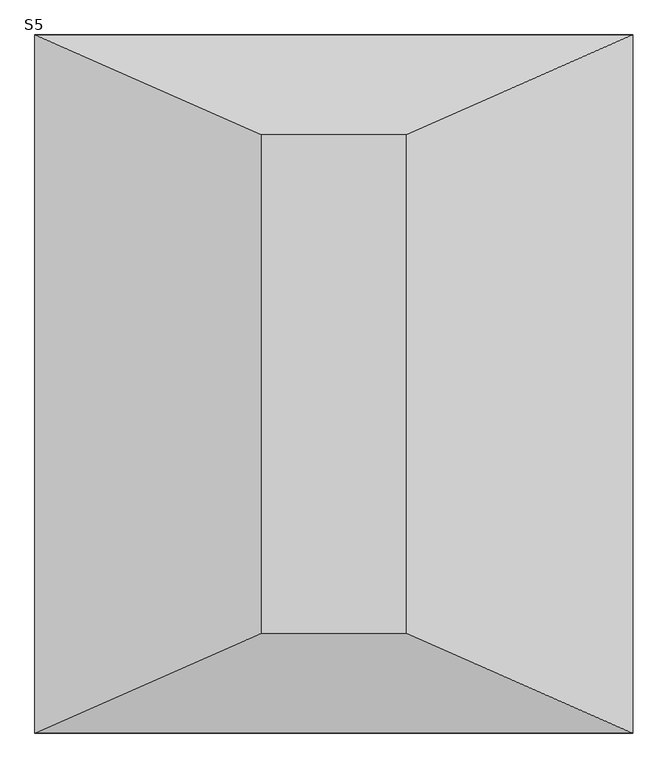
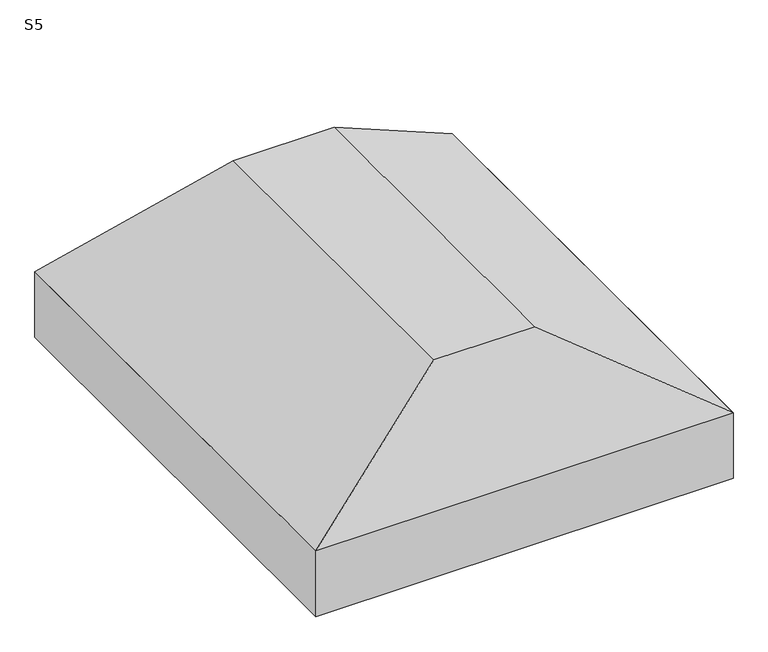
"""IFC4 building model written with IfcOpenShell, lengths in millimetres: fastener geometry, TQS - Sapata : S5."""

import ifcopenshell
import ifcopenshell.guid

model = None  # the IFC model being written
_history = None  # IfcOwnerHistory: only IFC2X3 demands one
_inside = {}  # id of a spatial element -> (the spatial element, [elements in it])
_under = {}  # id of a project, library or spatial element -> (it, [spatial elements below it])
_declared = {}  # id of a project -> (the project, [libraries it declares])
_typed = {}  # id of a type object -> (the type object, [elements of that type])
_made_of = {}  # id of a material, layer set ... -> (it, [elements and type objects made of it])


def new_model(schema):
    """Start an empty IFC model of exactly this schema.

    Asked for "IFC4X3", IfcOpenShell would pick the latest addendum, in which some entities
    have other attributes; the version numbers below select the first issue.
    IFC2X3 requires an IfcOwnerHistory on every rooted entity: one is made here for all.
    """
    global model, _history
    if schema == "IFC4X3":
        model = ifcopenshell.file(schema_version=(4, 3, 0, 0))
    else:
        model = ifcopenshell.file(schema=schema)
    _inside.clear()
    _under.clear()
    _declared.clear()
    _typed.clear()
    _made_of.clear()
    _history = None
    if model.schema == "IFC2X3":
        org = make("IfcOrganization", Name="unknown")
        user = make(
            "IfcPersonAndOrganization",
            ThePerson=make("IfcPerson", FamilyName="unknown"),
            TheOrganization=org,
        )
        app = make(
            "IfcApplication",
            ApplicationDeveloper=org,
            Version="unknown",
            ApplicationFullName="unknown",
            ApplicationIdentifier="unknown",
        )
        _history = make(
            "IfcOwnerHistory",
            OwningUser=user,
            OwningApplication=app,
            ChangeAction="ADDED",
            CreationDate=0,
        )
    return model


def make(cls, **values):
    """One entity of the class cls with the attributes given. An attribute that is None is left unset."""
    return model.create_entity(
        cls, **{name: value for name, value in values.items() if value is not None}
    )


def rooted(cls, **values):
    """An entity with a GlobalId (a new one), such as an element, a storey or a relation."""
    return make(cls, GlobalId=ifcopenshell.guid.new(), OwnerHistory=_history, **values)


def si_unit(unit_type, name, prefix=None):
    """IfcSIUnit, for example si_unit("LENGTHUNIT", "METRE", prefix="MILLI")."""
    return make("IfcSIUnit", UnitType=unit_type, Prefix=prefix, Name=name)


def assignment(units):
    """IfcUnitAssignment: the units of a project."""
    return None if units is None else make("IfcUnitAssignment", Units=units)


def point(xyz):
    """IfcCartesianPoint."""
    return None if xyz is None else make("IfcCartesianPoint", Coordinates=xyz)


def direction(xyz):
    """IfcDirection."""
    return None if xyz is None else make("IfcDirection", DirectionRatios=xyz)


def frame(location, z_axis=None, x_axis=None):
    """IfcAxis2Placement3D, a coordinate frame: its origin and axes. An axis left out is left unset."""
    return make(
        "IfcAxis2Placement3D",
        Location=point(location),
        Axis=direction(z_axis),
        RefDirection=direction(x_axis),
    )


def origin():
    """The frame at (0, 0, 0) with its axes left unset."""
    return frame((0.0, 0.0, 0.0))


def place(relative_to, where):
    """IfcLocalPlacement: puts the frame where relative to a parent placement (None: the world)."""
    return make(
        "IfcLocalPlacement", PlacementRelTo=relative_to, RelativePlacement=where
    )


def context(
    kind, dimensions, precision=None, world=None, true_north=None, identifier=None
):
    """IfcGeometricRepresentationContext, for example the 3D "Model" context."""
    return make(
        "IfcGeometricRepresentationContext",
        ContextIdentifier=identifier,
        ContextType=kind,
        CoordinateSpaceDimension=dimensions,
        Precision=precision,
        WorldCoordinateSystem=world,
        TrueNorth=true_north,
    )


def project(units=None, contexts=None):
    """IfcProject with its units and contexts."""
    return rooted(
        "IfcProject",
        Name="project",
        RepresentationContexts=contexts,
        UnitsInContext=assignment(units),
    )


def spatial(cls, under=None, at=None, **own):
    """A site, building, storey or space (cls), placed at a placement, below another one or the project."""
    s = rooted(cls, ObjectPlacement=at, **own)
    if under is not None:
        _under.setdefault(under.id(), (under, []))[1].append(s)
    return s


def polyline(points):
    """IfcPolyline through the points."""
    return make("IfcPolyline", Points=[point(p) for p in points])


def outline(outer, holes=None, kind="AREA"):
    """IfcArbitraryClosedProfileDef: a profile drawn as a closed curve; with holes, ...WithVoids."""
    if holes is None:
        return make("IfcArbitraryClosedProfileDef", ProfileType=kind, OuterCurve=outer)
    return make(
        "IfcArbitraryProfileDefWithVoids",
        ProfileType=kind,
        OuterCurve=outer,
        InnerCurves=holes,
    )


def extrude(swept, where, along, depth):
    """IfcExtrudedAreaSolid: the profile swept, set in the frame where, extruded along a direction by depth."""
    return make(
        "IfcExtrudedAreaSolid",
        SweptArea=swept,
        Position=where,
        ExtrudedDirection=direction(along),
        Depth=depth,
    )


def faces_of(points, faces, orient=None, outer=None):
    """IfcFace entities. A face is a list of loops; a loop is a list of indices into points, from 0.

    orient and outer hold one flag for each loop. By default every Orientation is true, the
    first loop of a face is its IfcFaceOuterBound and the others are IfcFaceBound.
    """
    made = []
    for i, loops in enumerate(faces):
        bounds = []
        for j, loop in enumerate(loops):
            is_outer = j == 0 if outer is None else outer[i][j]
            bounds.append(
                make(
                    "IfcFaceOuterBound" if is_outer else "IfcFaceBound",
                    Bound=make("IfcPolyLoop", Polygon=[points[k] for k in loop]),
                    Orientation=True if orient is None else orient[i][j],
                )
            )
        made.append(make("IfcFace", Bounds=bounds))
    return made


def faceted_brep(points, faces, orient=None, outer=None, voids=None):
    """IfcFacetedBrep: a solid bounded by flat faces; with voids (closed shells), ...WithVoids."""
    shared = [point(p) for p in points]
    hull = make("IfcClosedShell", CfsFaces=faces_of(shared, faces, orient, outer))
    if voids is None:
        return make("IfcFacetedBrep", Outer=hull)
    return make(
        "IfcFacetedBrepWithVoids",
        Outer=hull,
        Voids=[
            make(cls, CfsFaces=faces_of(shared, fs, o, b)) for cls, fs, o, b in voids
        ],
    )


def shape(context_of_items, identifier, shape_type, items):
    """IfcShapeRepresentation: the items that make up one representation, for example the "Body"."""
    return make(
        "IfcShapeRepresentation",
        ContextOfItems=context_of_items,
        RepresentationIdentifier=identifier,
        RepresentationType=shape_type,
        Items=items,
    )


def source(mapping_origin, context_of_items, identifier, shape_type, items):
    """IfcRepresentationMap: a shape defined once, which mapped items show again and again."""
    return make(
        "IfcRepresentationMap",
        MappingOrigin=mapping_origin,
        MappedRepresentation=shape(context_of_items, identifier, shape_type, items),
    )


def transform(
    local_origin,
    x_axis=None,
    y_axis=None,
    z_axis=None,
    scale=None,
    scale2=None,
    scale3=None,
    uniform=True,
):
    """IfcCartesianTransformationOperator3D, or its non-uniform kind. x_axis, y_axis, z_axis: its Axis1, 2, 3."""
    if uniform:
        return make(
            "IfcCartesianTransformationOperator3D",
            Axis1=direction(x_axis),
            Axis2=direction(y_axis),
            LocalOrigin=point(local_origin),
            Scale=scale,
            Axis3=direction(z_axis),
        )
    return make(
        "IfcCartesianTransformationOperator3DnonUniform",
        Axis1=direction(x_axis),
        Axis2=direction(y_axis),
        LocalOrigin=point(local_origin),
        Scale=scale,
        Axis3=direction(z_axis),
        Scale2=scale2,
        Scale3=scale3,
    )


def mapped(mapping_source, mapping_target):
    """IfcMappedItem: shows the shape of a source again, moved by a transform."""
    return make(
        "IfcMappedItem", MappingSource=mapping_source, MappingTarget=mapping_target
    )


def made_of(thing, what):
    """Note that an element or type object is made of a material, layer set ...; save() writes the relation."""
    if what is not None:
        _made_of.setdefault(what.id(), (what, []))[1].append(thing)
    return thing


def element(
    cls,
    number,
    at=None,
    inside=None,
    cuts=None,
    type_object=None,
    material=None,
    context=None,
    identifier="Body",
    shape_type=None,
    held_by="IfcProductDefinitionShape",
    body=None,
    shapes=None,
    **own,
):
    """One element of the class cls, such as IfcWall. Its Tag is "e" and its number.

    at: its placement. inside: the storey or other place that contains it. cuts: it is an
    opening in that element (IfcRelVoidsElement). A single representation is given by context,
    identifier, shape_type and body (its items); several are given by shapes. held_by: the class
    of the entity that holds the representations. save() writes the other relations.
    """
    e = rooted(cls, Tag="e%d" % number, ObjectPlacement=at, **own)
    if body is not None:
        shapes = [shape(context, identifier, shape_type, body)]
    if shapes is not None:
        e.Representation = make(held_by, Representations=shapes)
    if inside is not None:
        _inside.setdefault(inside.id(), (inside, []))[1].append(e)
    if cuts is not None:
        rooted(
            "IfcRelVoidsElement", RelatingBuildingElement=cuts, RelatedOpeningElement=e
        )
    if type_object is not None:
        _typed.setdefault(type_object.id(), (type_object, []))[1].append(e)
    return made_of(e, material)


def aggregate(whole, parts):
    """IfcRelAggregates: a whole, such as a stair, and the parts it consists of."""
    return rooted("IfcRelAggregates", RelatingObject=whole, RelatedObjects=parts)


def save(model, path):
    """Write the relations noted so far, then the file.

    IfcRelAggregates (storeys below a building ...), IfcRelContainedInSpatialStructure (elements
    in a storey), IfcRelDefinesByType, IfcRelAssociatesMaterial and IfcRelDeclares: one each for
    every whole, place, type object, material and project.
    """
    for whole, parts in _under.values():
        aggregate(whole, parts)
    for where, things in _inside.values():
        rooted(
            "IfcRelContainedInSpatialStructure",
            RelatedElements=things,
            RelatingStructure=where,
        )
    for kind, things in _typed.values():
        rooted("IfcRelDefinesByType", RelatedObjects=things, RelatingType=kind)
    for what, things in _made_of.values():
        rooted("IfcRelAssociatesMaterial", RelatedObjects=things, RelatingMaterial=what)
    for by, libraries in _declared.values():
        rooted("IfcRelDeclares", RelatingContext=by, RelatedDefinitions=libraries)
    model.write(path)


def s5_cab1d6eb(model_context):
    return source(origin(), model_context, "Body", "SolidModel", [
        faceted_brep([(-55.0, 300.0, 0.0), (-345.0, 300.0, 0.0), (-345.0, -700.0, 0.0), (-55.0, -700.0, 0.0), (400.0, 500.0, -300.0), (400.0, -900.0, -300.0), (-800.0, -900.0, -300.0), (-800.0, 500.0, -300.0)], [[[0, 1, 2, 3]], [[4, 5, 6, 7]], [[4, 7, 1, 0]], [[7, 6, 2, 1]], [[6, 5, 3, 2]], [[5, 4, 0, 3]]]),
        extrude(outline(polyline([(400.0, 500.0), (400.0, -900.0), (-800.0, -900.0), (-800.0, 500.0), (400.0, 500.0)])), frame((0.0, 0.0, -500.0), z_axis=(0.0, 0.0, 1.0), x_axis=(1.0, 0.0, 0.0)), (0.0, 0.0, 1.0), 200.0),
    ])


if __name__ == "__main__":
    model = new_model("IFC4")
    model_context = context("Model", 3, world=origin())
    ifc_project = project(units=[si_unit("LENGTHUNIT", "METRE", prefix="MILLI")], contexts=[model_context])
    site = spatial("IfcSite", under=ifc_project)
    building = spatial("IfcBuilding", under=site)
    placement = place(None, origin())
    s5_shape = s5_cab1d6eb(model_context)
    element("IfcFastener", 1, ObjectType="TQS - Sapata : S5", at=placement, inside=building, context=model_context, shape_type="MappedRepresentation", body=[
        mapped(s5_shape, transform((0.0, 0.0, 0.0), x_axis=(1.0, 0.0, 0.0), y_axis=(0.0, 1.0, 0.0), z_axis=(0.0, 0.0, 1.0))),
    ])
    save(model, "model.ifc")

# Revit data of these elements
# Type "TQS - Sapata : S5"
#   TY = 1.00 m
#   TX = 0.29 m
#   HS = 0.50 m
#   H0 = 0.20 m
#   EXCYABS = 0.70 m
#   EXCY = 0.00 m
#   EXCXABS = 0.60 m
#   EXCX = 0.00 m
#   DIMY = 1.40 m
#   DIMX = 1.20 m
#   Material estrutural = Concreto - Concreto concretado no local
#   Width = 0
#   Length = 0
# Element 1 (IfcFastener, "TQS - Sapata : S5")
#   Materials on its faces: "Concreto - Concreto concretado no local"
# Materials
#   "Concreto - Concreto concretado no local": class "Concreto", colour RGB 192 192 192, transparency 0
